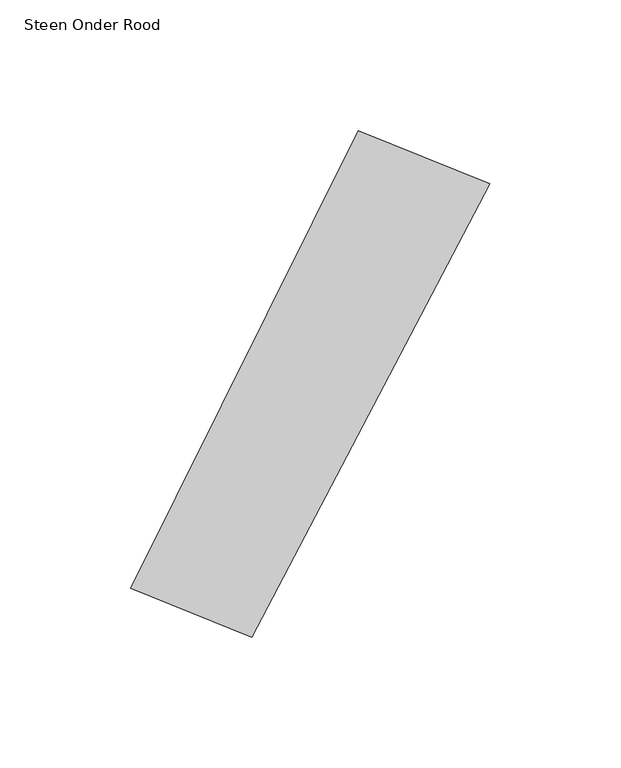
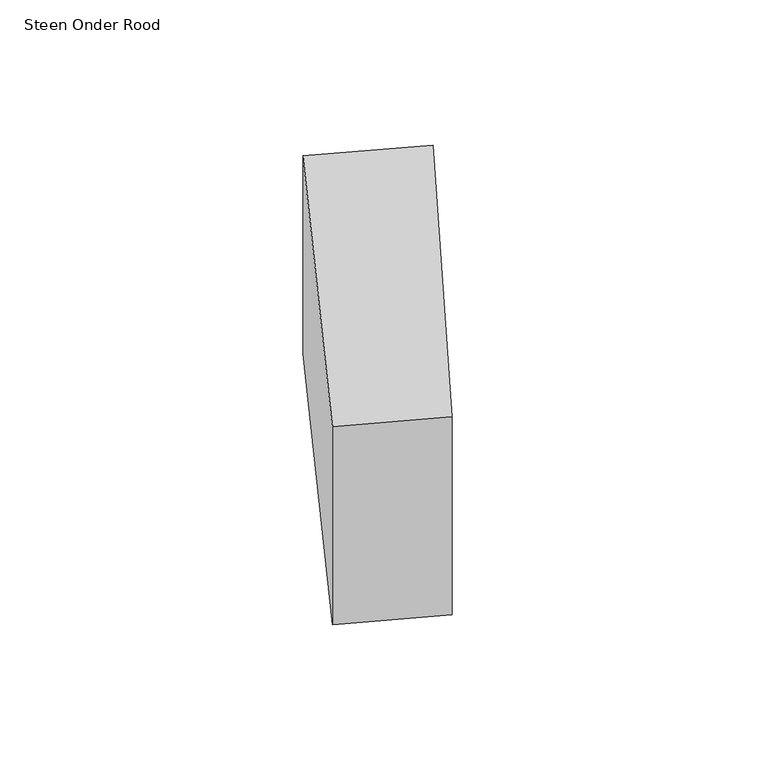
"""IFC4 building model written with IfcOpenShell, lengths in millimetres: proxy geometry, 00_GMA_steen_versie_4 : Steen Onder Rood."""

from ifc_helpers import new_model, si_unit, origin, origin_with_axes, place, context, project, spatial, polyline, outline, extrude, source, transform, mapped, element, save


def steen_onder_rood_ba3f12f9(model_context):
    return source(origin(), model_context, "Body", "SweptSolid", [
        extrude(outline(polyline([(145.3080509, 155.0219298), (54.2011876, -18.5127021), (7.8384531, 0.2088591), (94.9229116, 175.3588747), (145.3080509, 155.0219298)])), origin_with_axes(), (0.0, 0.0, 1.0), 100.0),
    ])


if __name__ == "__main__":
    model = new_model("IFC4")
    model_context = context("Model", 3, world=origin())
    ifc_project = project(units=[si_unit("LENGTHUNIT", "METRE", prefix="MILLI")], contexts=[model_context])
    site = spatial("IfcSite", under=ifc_project)
    building = spatial("IfcBuilding", under=site)
    placement = place(None, origin())
    steen_onder_rood_shape = steen_onder_rood_ba3f12f9(model_context)
    element("IfcBuildingElementProxy", 1, Name="00_GMA_steen_versie_4 : Steen Onder Rood", ObjectType="00_GMA_steen_versie_4 : Steen Onder Rood", at=placement, inside=building, context=model_context, shape_type="MappedRepresentation", body=[
        mapped(steen_onder_rood_shape, transform((0.0, 0.0, 0.0), x_axis=(1.0, 0.0, 0.0), y_axis=(0.0, 1.0, 0.0), z_axis=(0.0, 0.0, 1.0))),
    ])
    save(model, "model.ifc")

# Revit data of these elements
# Type "00_GMA_steen_versie_4 : Steen Onder Rood"
#   StootVoegHalfBoven [instance default] = 5 mm
#   StootVoegHalf [instance default] = 5 mm
#   StootVoegBreedteOnder = 10 mm
#   StootVoegBreedteBoven = 10 mm
#   Steendikte = 100 mm
#   LintVoegOnderHalf = 0 mm
#   LintVoegOnder = 0 mm
#   LintVoegBovenHalf = 5 mm
#   LintVoegBoven = 10 mm
#   materiaal = 21_steen_rood
#   MateriaalVoeg = none
#   Default Elevation = 0
# Element 1 (IfcBuildingElementProxy, "00_GMA_steen_versie_4 : Steen Onder Rood")
#   Materials on its faces: "21_steen_rood"
# Materials
#   "21_steen_rood": class "Unassigned", colour RGB 213 111 43, transparency 0, Cost = 0
